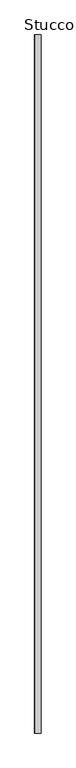
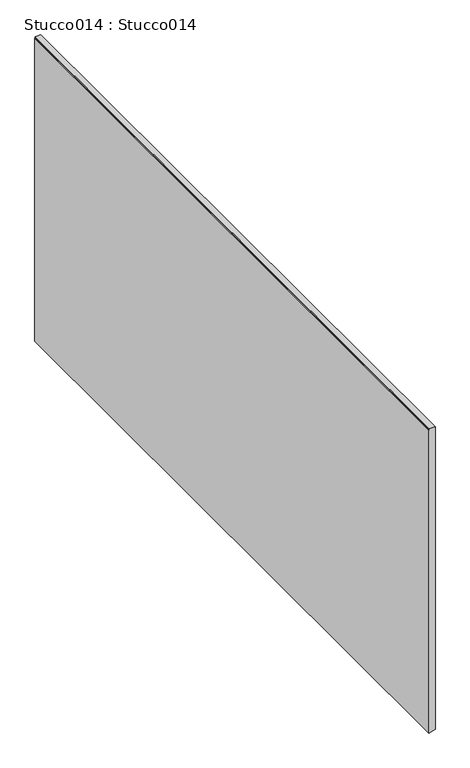
"""IFC4 building model written with IfcOpenShell, lengths in millimetres: proxy geometry, Stucco014 : Stucco014."""

from ifc_helpers import new_model, si_unit, frame, origin, place, context, project, spatial, polyline, outline, extrude, source, transform, mapped, element, save


def stucco014_stucco014_efddd258(model_context):
    return source(origin(), model_context, "Body", "SweptSolid", [
        extrude(outline(polyline([(33338.3622328, -9683.0763941), (34273.696139, -9683.0763941), (34273.696139, -9699.5865139), (34270.216339, -9699.5865139), (34270.216339, -9700.8565139), (33332.6487015, -9700.8565139), (33338.3622328, -9683.0763941)])), frame((0.0, 7982.1529359, 0.0), z_axis=(0.0, 1.0, 0.0), x_axis=(0.0, 0.0, 1.0)), (0.0, 0.0, 1.0), 2000.0),
    ])


if __name__ == "__main__":
    model = new_model("IFC4")
    model_context = context("Model", 3, world=origin())
    ifc_project = project(units=[si_unit("LENGTHUNIT", "METRE", prefix="MILLI")], contexts=[model_context])
    site = spatial("IfcSite", under=ifc_project)
    building = spatial("IfcBuilding", under=site)
    placement = place(None, origin())
    stucco014_stucco014_shape = stucco014_stucco014_efddd258(model_context)
    element("IfcBuildingElementProxy", 1, Name="Stucco014 : Stucco014", ObjectType="Stucco014 : Stucco014", at=placement, inside=building, context=model_context, shape_type="MappedRepresentation", body=[
        mapped(stucco014_stucco014_shape, transform((0.0, 0.0, 0.0), x_axis=(1.0, 0.0, 0.0), y_axis=(0.0, 1.0, 0.0), z_axis=(0.0, 0.0, 1.0))),
    ])
    save(model, "model.ifc")

# Revit data of these elements
# Type "Stucco014 : Stucco014"
#   NameOverride = "Stucco014"
# Element 1 (IfcBuildingElementProxy, "Stucco014 : Stucco014")
#   Materials on its faces: "7/8\" SMOOTH TROWEL EXTERIOR STUCCO"
# Materials
#   "7/8\" SMOOTH TROWEL EXTERIOR STUCCO": class "Unassigned", colour RGB 255 255 255, transparency 0, Cost = 0
